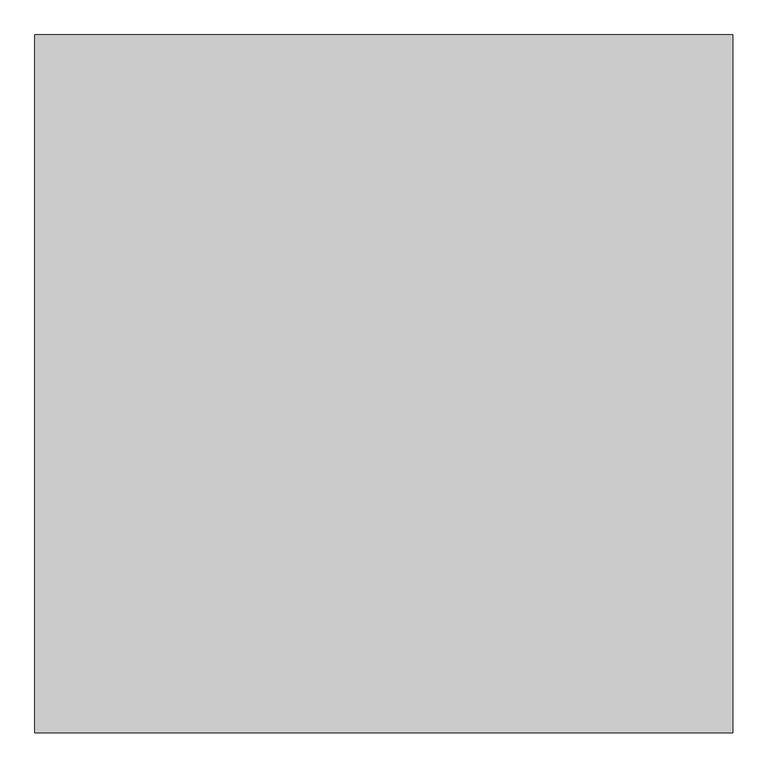
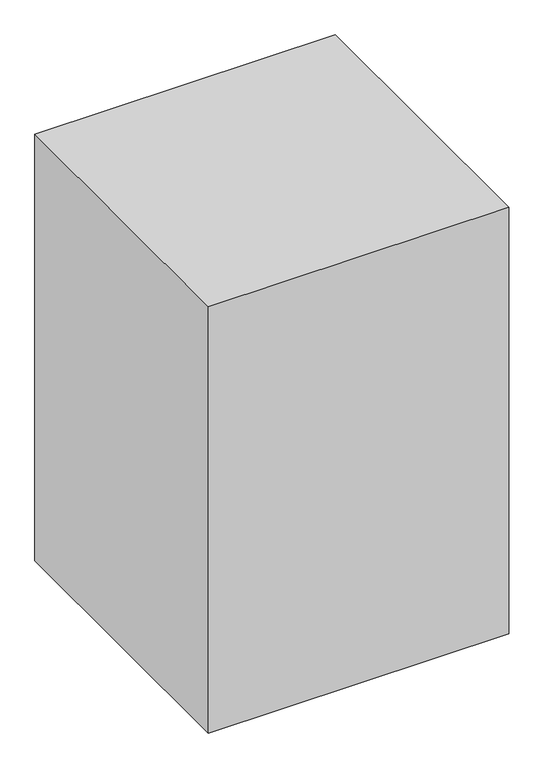
"""IFC4 building model written with IfcOpenShell, lengths in millimetres: proxy geometry, Space Planning Box_hec : Space Planning Box_hec."""

from ifc_helpers import new_model, si_unit, origin, origin_with_axes, place, context, project, spatial, polyline, outline, extrude, source, transform, mapped, element, save


def generic_models_7bff30ad(model_context):
    return source(origin(), model_context, "Body", "SweptSolid", [
        extrude(outline(polyline([(2000.0, 2000.0), (2000.0, -2000.0), (-2000.0, -2000.0), (-2000.0, 2000.0), (2000.0, 2000.0)])), origin_with_axes(), (0.0, 0.0, 1.0), 6000.0),
    ])


if __name__ == "__main__":
    model = new_model("IFC4")
    model_context = context("Model", 3, world=origin())
    ifc_project = project(units=[si_unit("LENGTHUNIT", "METRE", prefix="MILLI")], contexts=[model_context])
    site = spatial("IfcSite", under=ifc_project)
    building = spatial("IfcBuilding", under=site)
    placement = place(None, origin())
    generic_models_shape = generic_models_7bff30ad(model_context)
    element("IfcBuildingElementProxy", 1, Name="Space Planning Box_hec : Space Planning Box_hec", ObjectType="Space Planning Box_hec : Space Planning Box_hec", at=placement, inside=building, context=model_context, shape_type="MappedRepresentation", body=[
        mapped(generic_models_shape, transform((0.0, 0.0, 0.0), x_axis=(1.0, 0.0, 0.0), y_axis=(0.0, 1.0, 0.0), z_axis=(0.0, 0.0, 1.0))),
    ])
    save(model, "model.ifc")

# Revit data of these elements
# Type "Space Planning Box_hec : Space Planning Box_hec"
#   Type Comments = "..."
#   Room Name [instance default] = "?"
#   Interior Finish [instance default] = ""
#   Exterior Finish [instance default] = ""
#   Department [instance default] = ""
#   Assembly Code = "..."
#   Width [instance default] = 1524 mm
#   Program Area [instance default] = 0 m²
#   Length [instance default] = 1524 mm
#   Height [instance default] = 1524 mm
#   Area [instance default] = 2.32258 m²
#   Fill Color [instance default] = Cyan
#   Default Elevation = 0
# Element 1 (IfcBuildingElementProxy, "Space Planning Box_hec : Space Planning Box_hec")
#   Room Name = "Toilet (F)"
#   Interior Finish = "IF5"
#   Exterior Finish = "EF1"
#   Department = "AR"
#   Width = 4000 mm
#   Program Area = 72 m²
#   Length = 4000 mm
#   Height = 6000 mm
#   Area = 16 m²
#   Fill Color = Lavender
#   Materials on its faces: "Lavender"
# Materials
#   "Cyan": class "Generic", colour RGB 0 255 255, transparency 0.2, Cost = 0
#   "Lavender": class "Generic", colour RGB 186 85 211, transparency 0.2, Cost = 0
